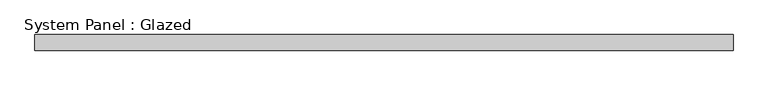
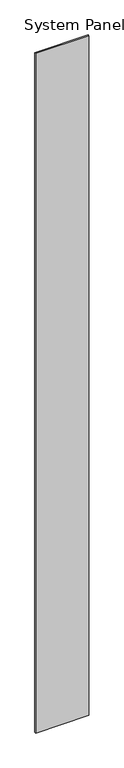
"""IFC4 building model written with IfcOpenShell, lengths in millimetres: plate geometry, System Panel : Glazed."""

from ifc_helpers import new_model, si_unit, origin, origin_with_axes, place, context, project, spatial, polyline, outline, extrude, source, transform, mapped, element, save


def system_panel_glazed_21f2c726(model_context):
    return source(origin(), model_context, "Body", "SweptSolid", [
        extrude(outline(polyline([(553.4450969, 19.05), (-553.4450969, 19.05), (-553.4450969, 44.45), (553.4450969, 44.45), (553.4450969, 19.05)])), origin_with_axes(), (0.0, 0.0, 1.0), 14960.6),
    ])


if __name__ == "__main__":
    model = new_model("IFC4")
    model_context = context("Model", 3, world=origin())
    ifc_project = project(units=[si_unit("LENGTHUNIT", "METRE", prefix="MILLI")], contexts=[model_context])
    site = spatial("IfcSite", under=ifc_project)
    building = spatial("IfcBuilding", under=site)
    placement = place(None, origin())
    system_panel_glazed_shape = system_panel_glazed_21f2c726(model_context)
    element("IfcPlate", 1, ObjectType="System Panel : Glazed", at=placement, inside=building, context=model_context, shape_type="MappedRepresentation", body=[
        mapped(system_panel_glazed_shape, transform((0.0, 0.0, 0.0), x_axis=(1.0, 0.0, 0.0), y_axis=(0.0, 1.0, 0.0), z_axis=(0.0, 0.0, 1.0))),
    ])
    save(model, "model.ifc")

# Revit data of these elements
# Type "System Panel : Glazed"
#   Construction Type Id = "GSP4R"
#   Analytic Construction = "1/8 in Pilkington single glazing"
#   Visual Light Transmittance = 0.9
#   Solar Heat Gain Coefficient = 0.86
#   Heat Transfer Coefficient (U) = 1.18115 BTU/(h·ft²·°F)
#   Define Thermal Properties by = 1
# Element 1 (IfcPlate, "System Panel : Glazed")
#   Materials on its faces: "Glass"
# Materials
#   "Glass": class "Glass", colour RGB 0 128 192, transparency 0.75, Description = "Soda Lime Glass", Cost = 0
